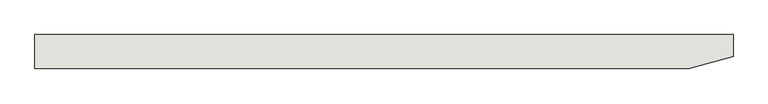
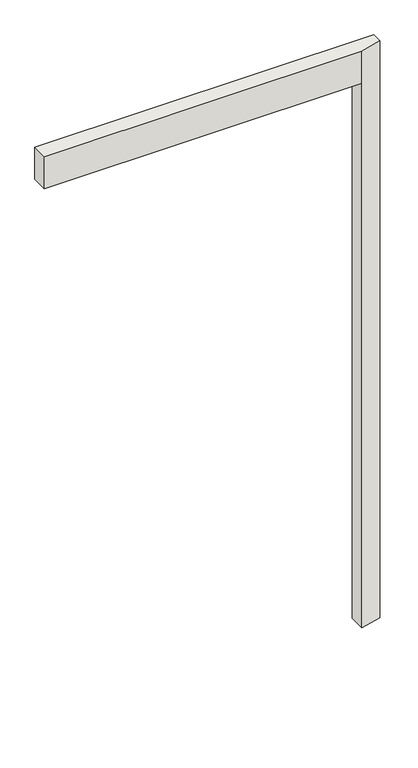
"""IFC4 building model written with IfcOpenShell, lengths in millimetres: wall geometry, 0_3d_modell."""

from ifc_helpers import new_model, si_unit, origin, place, context, project, spatial, faceted_brep, source, transform, mapped, element, save


def wall_20571731(model_context):
    return source(origin(), model_context, "Body", "Brep", [
        faceted_brep([(0.0, 78.0, 2720.0), (1500.0, 78.0, 2720.0), (1500.0, 0.0, 2720.0), (0.0, 0.0, 2720.0), (1500.0, 78.0, 0.0), (1500.0, 0.0, 0.0), (0.0, 78.0, 2880.0), (1600.0, 78.0, 2880.0), (1600.0, 78.0, 0.0), (0.0, 0.0, 2880.0), (1600.0, 28.0, 0.0), (1600.0, 28.0, 2880.0), (1500.0, 0.0, 2880.0)], [[[0, 1, 2, 3]], [[1, 4, 5, 2]], [[4, 1, 0, 6, 7, 8]], [[0, 3, 9, 6]], [[10, 8, 7, 11]], [[5, 10, 11, 12, 2]], [[3, 2, 12, 9]], [[9, 12, 11, 7, 6]], [[5, 4, 8, 10]]]),
    ])


if __name__ == "__main__":
    model = new_model("IFC4")
    model_context = context("Model", 3, world=origin())
    ifc_project = project(units=[si_unit("LENGTHUNIT", "METRE", prefix="MILLI")], contexts=[model_context])
    site = spatial("IfcSite", under=ifc_project)
    building = spatial("IfcBuilding", under=site)
    placement = place(None, origin())
    wall_shape = wall_20571731(model_context)
    element("IfcWall", 1, ObjectType="0_3d_modell", at=placement, inside=building, context=model_context, shape_type="MappedRepresentation", body=[
        mapped(wall_shape, transform((0.0, 0.0, 0.0), x_axis=(1.0, 0.0, 0.0), y_axis=(0.0, 1.0, 0.0), z_axis=(0.0, 0.0, 1.0))),
    ])
    save(model, "model.ifc")

# Revit data of these elements
# Element 1 (IfcWall, "0_3d_modell")
#   Materials on its faces: "glas"
# Materials
#   "glas": class "Unassigned", colour RGB 250 253 254, transparency 0.95
